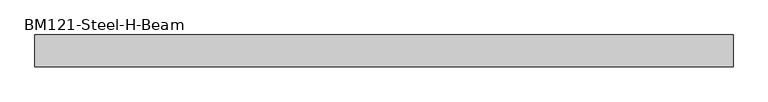
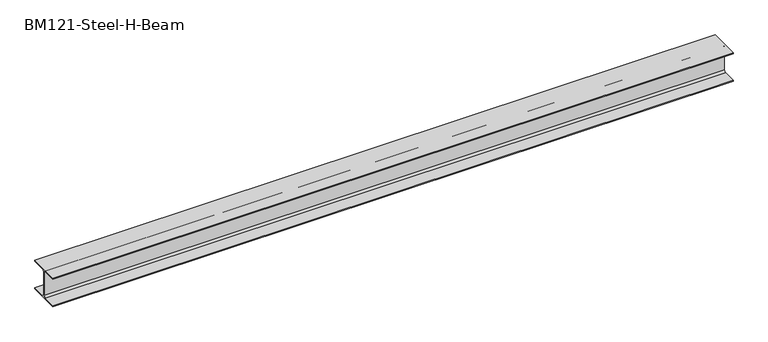
"""IFC4 building model written with IfcOpenShell, lengths in millimetres: beam geometry, BM121-Steel-H-Beam : BM121_H-294×302x12x12."""

from ifc_helpers import new_model, si_unit, point, frame, frame_2d, origin, place, context, project, spatial, polyline, circle_curve, trimmed, segment, composite_curve, outline, extrude, source, transform, mapped, element, save


def bm121_steel_h_beam_e4b020da(model_context):
    return source(origin(), model_context, "Body", "SweptSolid", [
        extrude(outline(composite_curve([segment(polyline([(-151.0, 147.0), (151.0, 147.0), (151.0, 135.0), (24.0, 135.0)]), True, "CONTINUOUS"), segment(trimmed(circle_curve(frame_2d((24.0, 117.0)), 18.0), [point((24.0, 135.0))], [point((6.0, 117.0))], True, "CARTESIAN"), True, "CONTINUOUS"), segment(polyline([(6.0, 117.0), (6.0, -117.0)]), True, "CONTINUOUS"), segment(trimmed(circle_curve(frame_2d((24.0, -117.0)), 18.0), [point((6.0, -117.0))], [point((24.0, -135.0))], True, "CARTESIAN"), True, "CONTINUOUS"), segment(polyline([(24.0, -135.0), (151.0, -135.0), (151.0, -147.0), (-151.0, -147.0), (-151.0, -135.0), (-24.0, -135.0)]), True, "CONTINUOUS"), segment(trimmed(circle_curve(frame_2d((-24.0, -117.0)), 18.0), [point((-24.0, -135.0))], [point((-6.0, -117.0))], True, "CARTESIAN"), True, "CONTINUOUS"), segment(polyline([(-6.0, -117.0), (-6.0, 117.0)]), True, "CONTINUOUS"), segment(trimmed(circle_curve(frame_2d((-24.0, 117.0)), 18.0), [point((-6.0, 117.0))], [point((-24.0, 135.0))], True, "CARTESIAN"), True, "CONTINUOUS"), segment(polyline([(-24.0, 135.0), (-151.0, 135.0), (-151.0, 147.0)]), True, "CONTINUOUS")], self_intersect=False)), frame((-3270.6243373, 0.0, 0.0), z_axis=(1.0, 0.0, 0.0), x_axis=(0.0, 1.0, 0.0)), (0.0, 0.0, 1.0), 6592.2),
    ])


if __name__ == "__main__":
    model = new_model("IFC4")
    model_context = context("Model", 3, world=origin())
    ifc_project = project(units=[si_unit("LENGTHUNIT", "METRE", prefix="MILLI")], contexts=[model_context])
    site = spatial("IfcSite", under=ifc_project)
    building = spatial("IfcBuilding", under=site)
    placement = place(None, origin())
    bm121_steel_h_beam_shape = bm121_steel_h_beam_e4b020da(model_context)
    element("IfcBeam", 1, ObjectType="BM121-Steel-H-Beam : BM121_H-294×302x12x12", at=placement, inside=building, context=model_context, shape_type="MappedRepresentation", body=[
        mapped(bm121_steel_h_beam_shape, transform((0.0, 0.0, 0.0), x_axis=(1.0, 0.0, 0.0), y_axis=(0.0, 1.0, 0.0), z_axis=(0.0, 0.0, 1.0))),
    ])
    save(model, "model.ifc")

# Revit data of these elements
# Type "BM121-Steel-H-Beam : BM121_H-294×302x12x12"
#   tw = 12 mm
#   tf = 12 mm
#   r = 18 mm
#   bf = 302 mm
#   Unit Weight = 84.50 kg/m
#   Surface Area = 1.7411 m²/m
#   Length [instance default] = 3000 mm
#   H = 294 mm
#   Sectional Area = 10770.0 cm²
